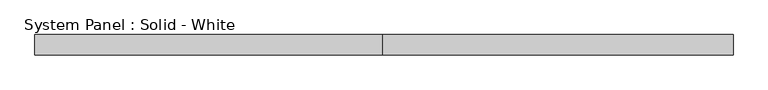
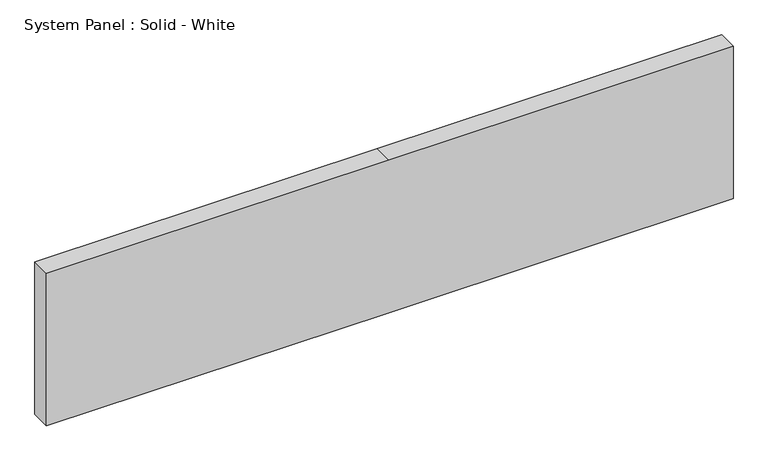
"""IFC4 building model written with IfcOpenShell, lengths in millimetres: plate geometry, System Panel : Solid - White."""

from ifc_helpers import new_model, si_unit, frame, origin, place, context, project, spatial, polyline, outline, extrude, source, transform, mapped, element, save


def system_panel_solid_white_9f65361e(model_context):
    return source(origin(), model_context, "Body", "SweptSolid", [
        extrude(outline(polyline([(0.0, -1094.2054237), (0.0, -3.6091526), (0.0, 1094.2054237), (514.35, 1094.2054237), (514.35, -3.6091526), (514.35, -1094.2054237), (0.0, -1094.2054237)])), frame((0.0, -19.05, 0.0), z_axis=(0.0, 1.0, 0.0), x_axis=(0.0, 0.0, 1.0)), (0.0, 0.0, 1.0), 63.5),
    ])


if __name__ == "__main__":
    model = new_model("IFC4")
    model_context = context("Model", 3, world=origin())
    ifc_project = project(units=[si_unit("LENGTHUNIT", "METRE", prefix="MILLI")], contexts=[model_context])
    site = spatial("IfcSite", under=ifc_project)
    building = spatial("IfcBuilding", under=site)
    placement = place(None, origin())
    system_panel_solid_white_shape = system_panel_solid_white_9f65361e(model_context)
    element("IfcPlate", 1, ObjectType="System Panel : Solid - White", at=placement, inside=building, context=model_context, shape_type="MappedRepresentation", body=[
        mapped(system_panel_solid_white_shape, transform((0.0, 0.0, 0.0), x_axis=(1.0, 0.0, 0.0), y_axis=(0.0, 1.0, 0.0), z_axis=(0.0, 0.0, 1.0))),
    ])
    save(model, "model.ifc")

# Revit data of these elements
# Element 1 (IfcPlate, "System Panel : Solid - White")
#   Materials on its faces: "White Panel"
# Materials
#   "White Panel": class "Unassigned", colour RGB 255 255 255, transparency 0
